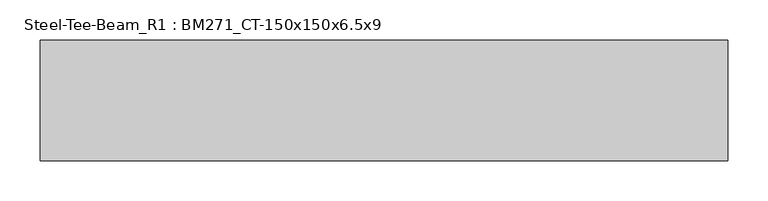
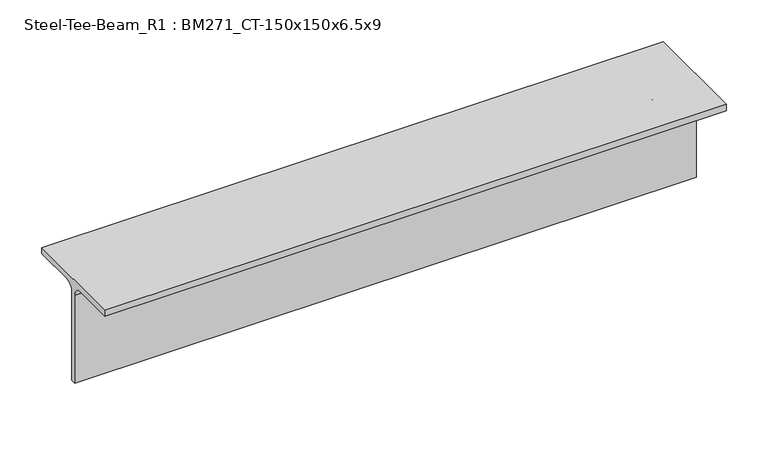
"""IFC4 building model written with IfcOpenShell, lengths in millimetres: member geometry, Steel-Tee-Beam_R1 : BM271_CT-150x150x6.5x9."""

from ifc_helpers import new_model, si_unit, point, frame, frame_2d, origin, place, context, project, spatial, polyline, circle_curve, trimmed, segment, composite_curve, outline, extrude, source, transform, mapped, element, save


def steel_tee_beam_r1_bm271_ct_150x150x6_5x9_b6a32e11(model_context):
    return source(origin(), model_context, "Body", "SweptSolid", [
        extrude(outline(composite_curve([segment(polyline([(-75.0, 75.0), (75.0, 75.0), (75.0, 66.0), (16.25, 66.0)]), True, "CONTINUOUS"), segment(trimmed(circle_curve(frame_2d((16.25, 53.0)), 13.0), [point((16.25, 66.0))], [point((3.25, 53.0))], True, "CARTESIAN"), True, "CONTINUOUS"), segment(polyline([(3.25, 53.0), (3.25, -75.0), (-3.25, -75.0), (-3.25, 53.0)]), True, "CONTINUOUS"), segment(trimmed(circle_curve(frame_2d((-16.25, 53.0)), 13.0), [point((-3.25, 53.0))], [point((-16.25, 66.0))], True, "CARTESIAN"), True, "CONTINUOUS"), segment(polyline([(-16.25, 66.0), (-75.0, 66.0), (-75.0, 75.0)]), True, "CONTINUOUS")], self_intersect=False)), frame((-500.0, 0.0, 0.0), z_axis=(1.0, 0.0, 0.0), x_axis=(0.0, 1.0, 0.0)), (0.0, 0.0, 1.0), 856.1687518),
    ])


if __name__ == "__main__":
    model = new_model("IFC4")
    model_context = context("Model", 3, world=origin())
    ifc_project = project(units=[si_unit("LENGTHUNIT", "METRE", prefix="MILLI")], contexts=[model_context])
    site = spatial("IfcSite", under=ifc_project)
    building = spatial("IfcBuilding", under=site)
    placement = place(None, origin())
    steel_tee_beam_r1_bm271_ct_150x150x6_5x9_shape = steel_tee_beam_r1_bm271_ct_150x150x6_5x9_b6a32e11(model_context)
    element("IfcMember", 1, ObjectType="Steel-Tee-Beam_R1 : BM271_CT-150x150x6.5x9", at=placement, inside=building, context=model_context, shape_type="MappedRepresentation", body=[
        mapped(steel_tee_beam_r1_bm271_ct_150x150x6_5x9_shape, transform((0.0, 0.0, 0.0), x_axis=(1.0, 0.0, 0.0), y_axis=(0.0, 1.0, 0.0), z_axis=(0.0, 0.0, 1.0))),
    ])
    save(model, "model.ifc")

# Revit data of these elements
# Type "Steel-Tee-Beam_R1 : BM271_CT-150x150x6.5x9"
#   Keynote = "CT-150x150x6.5x9"
#   Surface Area = 0.588841 m²/m
#   Section Area = 23.3904 cm²
#   Mass per Unit Length = 18.3614 kg/m
#   Length [instance default] = 1.5240 m
#   bf = 0.1500 m
#   d = 0.1500 m
#   k = 0.0220 m
#   r = 0.0130 m
#   tf = 0.0090 m
#   tw = 0.0065 m
#   hec_material4 [instance default] = none
#   hec_material3 [instance default] = none
#   hec_material2 [instance default] = none
#   hec_material1 [instance default] = none
#   Structural Material [instance default] = Steel, 45-345
#   Assembly Code = ""
# Element 1 (IfcMember, "Steel-Tee-Beam_R1 : BM271_CT-150x150x6.5x9")
#   Structural Material = none
# Materials
#   "Steel, 45-345": class "Metal", colour RGB 189 187 185, transparency 0, Description = "Steel 345 MPa", Cost = 0
